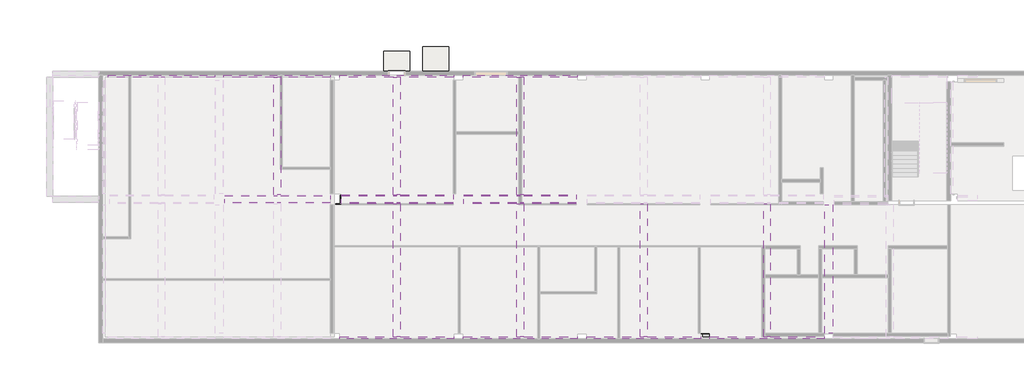
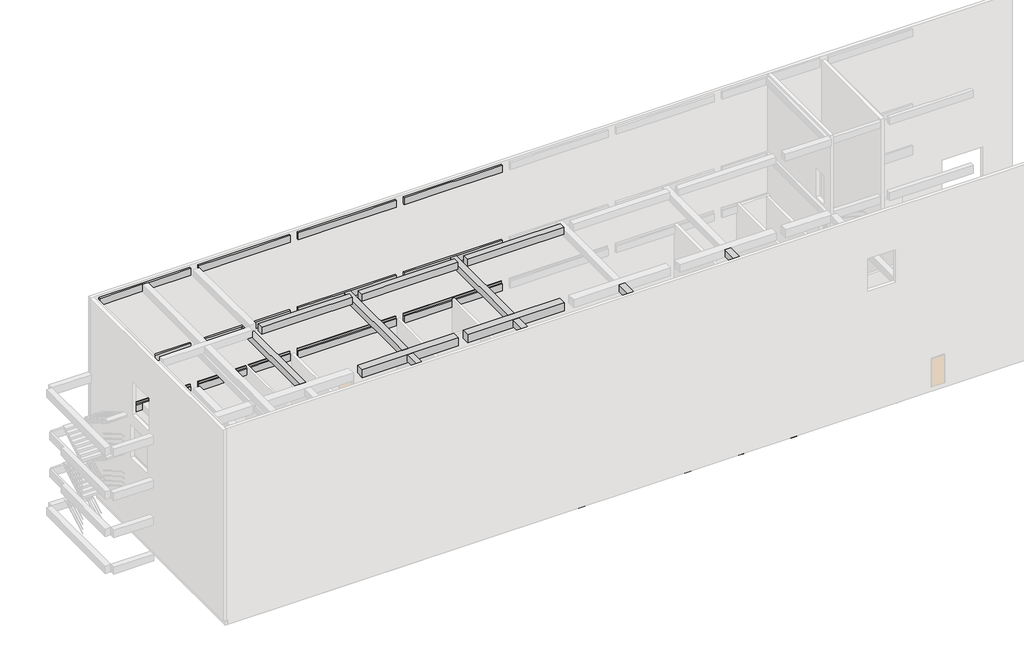
# One storey, part 3 of 5: 54 beams, 2 slabs.
# Revit data of these elements (continued)
# Room at (49621.297, 12708.408) mm, phase "New Construction", upper level "TOC", upper offset 9000 mm, lower offset 0 mm (continued)
#   H_Wall-Base Material-2 = ""
#   H_Wall-Base Material-3 = ""
#   H_Floor-Base Material-1 = "Concrete Slab"
#   H_Floor-Base Material-2 = ""
#   H_Floor-Base Material-3 = "Screed"
#   H_Floor-Base Material-4 = "Waterproof Membrane"
#   H_Floor-Base Material-5 = "Ceramic Tile"
#   H_Floor Finish-1 = "Ceramic Tile"
#   H_Floor Finish-2 = ""
#   H_Floor Finish Remark = ""
#   H_Skirt Base Material = "Same as Wall"
#   H_Skirt-Base Material-1 = ""
#   H_Skirt-Base Material-2 = ""
#   H_Skirt-Base Material-3 = ""
#   H_Skirt-Base Material-4 = ""
#   H_Skirt-Base Material-5 = ""
#   H_Skirt Finish-1 = "Acrylic Emulsion Paint"
#   H_Skirt Finish-2 = ""
#   H_Skirt Finish Remark = ""
#   H_Wall Finish Style Name = "Glazed Ceramic Tile (≤C.H+100) / No Paint (>C.H+100)"
#   H_Wall Base Material = "Masonry Wall / Waterproof Membrane"
#   H_Wall-Base Material-4 = "Waterproof Membrane"
#   H_Wall-Base Material-5 = "Glazed Ceramic Tile"
#   H_Wall Finish-1 = "Glazed Ceramic Tile"
#   H_Wall Finish-2 = ""
#   H_Wall Finish Remark = "Below Suspended Ceiling\nGlazed Ceramic Tile(≤C.H+100) + Waterproofing Membrane / No Paint (>C.H+100)"
#   H_Ceiling Finish Style Name = "Suspended Moisture Resistant Tiled Ceiling (T-Bar)"
#   H_Ceiling Base Material = "Concrete Slab / Fair Faced Concrete"
#   H_Ceiling-Base Material-1 = "(Concrete Slab)"
#   H_Ceiling-Base Material-2 = "(Fair Faced Concrete)"
#   H_Ceiling-Base Material-3 = ""
#   H_Ceiling-Base Material-4 = ""
#   H_Ceiling-Base Material-5 = "Moisture Resistant Tiled Ceiling System (T-Bar)"
#   H_Ceiling Finish-1 = "Moisture Resistant Tiled Ceiling System (T-Bar)"
#   H_Ceiling Finish-2 = ""
#   H_Ceiling Finish Remark = "600x600\nT bar"
#   H_Room W = 2700 mm
#   H_Room L = 1400 mm
#   H_Room H or CH = 9000 mm
#   Floor Finish Style No = none
#   Skirt Finish Style No = none
#   Wall Finish Style No = W32F
#   Ceiling Finish Style No = C96B
# Room at (52871.108, 13591.136) mm, phase "New Construction", upper level "TOC", upper offset 9000 mm, lower offset 0 mm
#   Comments = ""
#   Number = "110"
#   Name = "STAIRCASE"
#   H_Floor Finish Style Name = "Vinyl Tile"
#   H_Floor Base Material = "Concrete Slab / Steel Trowel Finish"
#   H_Wall-Base Material-1 = "Concrete Wall"
#   H_Skirt Finish Style Name = "Coved Vinyl Tile"
#   H_Wall-Base Material-2 = "(Fair Faced Concrete)"
#   H_Wall-Base Material-3 = ""
#   H_Floor-Base Material-1 = "Concrete Slab"
#   H_Floor-Base Material-2 = "Steel Trowel Finish"
#   H_Floor-Base Material-3 = ""
#   H_Floor-Base Material-4 = ""
#   H_Floor-Base Material-5 = "Vinyl Tile"
#   H_Floor Finish-1 = "Vinyl Tile"
#   H_Floor Finish-2 = ""
#   H_Floor Finish Remark = ""
#   H_Skirt Base Material = "Same as Wall"
#   H_Skirt-Base Material-1 = ""
#   H_Skirt-Base Material-2 = ""
#   H_Skirt-Base Material-3 = ""
#   H_Skirt-Base Material-4 = ""
#   H_Skirt-Base Material-5 = ""
#   H_Skirt Finish-1 = "Vinyl Tile"
#   H_Skirt Finish-2 = ""
#   H_Skirt Finish Remark = "Vinyl Tile = PVC Tile (polyvinyl chloride)"
#   H_Wall Finish Style Name = "Water Emulsion Paint"
#   H_Wall Base Material = "Concrete Wall / Fair Faced Concrete"
#   H_Wall-Base Material-4 = ""
#   H_Wall-Base Material-5 = ""
#   H_Wall Finish-1 = "Water Emulsion Paint"
#   H_Wall Finish-2 = ""
#   H_Wall Finish Remark = ""
#   H_Ceiling Finish Style Name = "Water Emulsion Paint"
#   H_Ceiling Base Material = "Concrete Slab / Fair Faced Concrete"
#   H_Ceiling-Base Material-1 = "(Concrete Slab)"
#   H_Ceiling-Base Material-2 = ""
#   H_Ceiling-Base Material-3 = ""
#   H_Ceiling-Base Material-4 = ""
#   H_Ceiling-Base Material-5 = ""
#   H_Ceiling Finish-1 = "Water Emulsion Paint"
#   H_Ceiling Finish-2 = ""
#   H_Ceiling Finish Remark = ""
#   H_Room W = 2000 mm
#   H_Room L = 8000 mm
#   H_Room H or CH = 9000 mm
#   Floor Finish Style No = none
#   Skirt Finish Style No = none
#   Wall Finish Style No = W02A
#   Ceiling Finish Style No = C02
# Room at (56962.839, 14779.531) mm, phase "New Construction", upper level "TOC", upper offset 9000 mm, lower offset 0 mm
#   Comments = ""
#   Number = "124"
#   Name = "F.O TANK ROOM"
#   H_Floor Finish Style Name = "Non-Slip Epoxy Paint"
#   H_Floor Base Material = "Concrete Slab / Steel Trowel Finish"
#   H_Wall-Base Material-1 = "Masonry Wall"
#   H_Skirt Finish Style Name = "Epoxy Paint"
#   H_Wall-Base Material-2 = ""
#   H_Wall-Base Material-3 = "Plastering"
#   H_Floor-Base Material-1 = "Concrete Slab"
#   H_Floor-Base Material-2 = "Steel Trowel Finish"
#   H_Floor-Base Material-3 = ""
#   H_Floor-Base Material-4 = ""
#   H_Floor-Base Material-5 = ""
#   H_Floor Finish-1 = "Epoxy Paint"
#   H_Floor Finish-2 = ""
#   H_Floor Finish Remark = "*WM 기준 확인 필요 Epoxy Paint \n(용제형, 0.1mm 이하) : epoxy resin + polyamine hardener(경화제)"
#   H_Skirt Base Material = "Same as Wall"
#   H_Skirt-Base Material-1 = ""
#   H_Skirt-Base Material-2 = ""
#   H_Skirt-Base Material-3 = ""
#   H_Skirt-Base Material-4 = ""
#   H_Skirt-Base Material-5 = ""
#   H_Skirt Finish-1 = "Epoxy Paint"
#   H_Skirt Finish-2 = ""
#   H_Skirt Finish Remark = "SACE"
#   H_Wall Finish Style Name = "Water Emulsion Paint"
#   H_Wall Base Material = "Masonry Wall / Cement Plaster"
#   H_Wall-Base Material-4 = ""
#   H_Wall-Base Material-5 = ""
#   H_Wall Finish-1 = ""
#   H_Wall Finish-2 = ""
#   H_Wall Finish Remark = ""
#   H_Ceiling Finish Style Name = "Water Emulsion Paint"
#   H_Ceiling Base Material = "Concrete Slab / Fair Faced Concrete"
#   H_Ceiling-Base Material-1 = "(Concrete Slab)"
#   H_Ceiling-Base Material-2 = ""
#   H_Ceiling-Base Material-3 = ""
#   H_Ceiling-Base Material-4 = ""
#   H_Ceiling-Base Material-5 = ""
#   H_Ceiling Finish-1 = "Water Emulsion Paint"
#   H_Ceiling Finish-2 = ""
#   H_Ceiling Finish Remark = ""
#   H_Room W = 3800 mm
#   H_Room L = 8400 mm
#   H_Room H or CH = 9000 mm
#   Floor Finish Style No = none
#   Skirt Finish Style No = none
#   Wall Finish Style No = W02B
#   Ceiling Finish Style No = C02
# Room at (61954.58, 4867.401) mm, phase "New Construction", upper level "TOC", upper offset 9000 mm, lower offset 0 mm
#   Comments = ""
#   Number = "125"
#   Name = "HVAC ROOM"
#   H_Floor Finish Style Name = "Non-Slip Epoxy Paint"
#   H_Floor Base Material = "Concrete Slab / Steel Trowel Finish"
#   H_Wall-Base Material-1 = "Masonry Wall"
#   H_Skirt Finish Style Name = "Epoxy Paint"
#   H_Wall-Base Material-2 = ""
#   H_Wall-Base Material-3 = "Plastering"
#   H_Floor-Base Material-1 = "Concrete Slab"
#   H_Floor-Base Material-2 = "Steel Trowel Finish"
#   H_Floor-Base Material-3 = ""
#   H_Floor-Base Material-4 = ""
#   H_Floor-Base Material-5 = ""
#   H_Floor Finish-1 = "Epoxy Paint"
#   H_Floor Finish-2 = ""
#   H_Floor Finish Remark = "*WM 기준 확인 필요 Epoxy Paint \n(용제형, 0.1mm 이하) : epoxy resin + polyamine hardener(경화제)"
#   H_Skirt Base Material = "Same as Wall"
#   H_Skirt-Base Material-1 = ""
#   H_Skirt-Base Material-2 = ""
#   H_Skirt-Base Material-3 = ""
#   H_Skirt-Base Material-4 = ""
#   H_Skirt-Base Material-5 = ""
#   H_Skirt Finish-1 = "Epoxy Paint"
#   H_Skirt Finish-2 = ""
#   H_Skirt Finish Remark = "SACE"
#   H_Wall Finish Style Name = "Water Emulsion Paint"
#   H_Wall Base Material = "Masonry Wall / Cement Plaster"
#   H_Wall-Base Material-4 = ""
#   H_Wall-Base Material-5 = ""
#   H_Wall Finish-1 = ""
#   H_Wall Finish-2 = ""
#   H_Wall Finish Remark = ""
#   H_Room W = 3600 mm
#   H_Room L = 4100 mm
#   H_Room H or CH = 9000 mm
#   Floor Finish Style No = none
#   Skirt Finish Style No = none
#   Wall Finish Style No = W02B
# Room at (52877.947, 3986.832) mm, phase "New Construction", upper level "TOC", upper offset 9000 mm, lower offset 0 mm
#   Comments = ""
#   Number = "122"
#   Name = "CYLINDER ROOM (HFC-23)"
#   H_Floor Finish Style Name = "Non-Slip Epoxy Paint"
#   H_Floor Base Material = "Concrete Slab / Steel Trowel Finish"
#   H_Wall-Base Material-1 = "Masonry Wall"
#   H_Skirt Finish Style Name = "Epoxy Paint"
#   H_Wall-Base Material-2 = ""
#   H_Wall-Base Material-3 = "Plastering"
#   H_Floor-Base Material-1 = "Concrete Slab"
#   H_Floor-Base Material-2 = "Steel Trowel Finish"
#   H_Floor-Base Material-3 = ""
#   H_Floor-Base Material-4 = ""
#   H_Floor-Base Material-5 = ""
#   H_Floor Finish-1 = "Epoxy Paint"
#   H_Floor Finish-2 = ""
#   H_Floor Finish Remark = "*WM 기준 확인 필요 Epoxy Paint \n(용제형, 0.1mm 이하) : epoxy resin + polyamine hardener(경화제)"
#   H_Skirt Base Material = "Same as Wall"
#   H_Skirt-Base Material-1 = ""
#   H_Skirt-Base Material-2 = ""
#   H_Skirt-Base Material-3 = ""
#   H_Skirt-Base Material-4 = ""
#   H_Skirt-Base Material-5 = ""
#   H_Skirt Finish-1 = "Epoxy Paint"
#   H_Skirt Finish-2 = ""
#   H_Skirt Finish Remark = "SACE"
#   H_Wall Finish Style Name = "Water Emulsion Paint"
#   H_Wall Base Material = "Masonry Wall / Cement Plaster"
#   H_Wall-Base Material-4 = ""
#   H_Wall-Base Material-5 = ""
#   H_Wall Finish-1 = ""
#   H_Wall Finish-2 = ""
#   H_Wall Finish Remark = ""
#   H_Ceiling Finish Style Name = "Water Emulsion Paint"
#   H_Ceiling Base Material = "Concrete Slab / Fair Faced Concrete"
#   H_Ceiling-Base Material-1 = "(Concrete Slab)"
#   H_Ceiling-Base Material-2 = ""
#   H_Ceiling-Base Material-3 = ""
#   H_Ceiling-Base Material-4 = ""
#   H_Ceiling-Base Material-5 = ""
#   H_Ceiling Finish-1 = "Water Emulsion Paint"
#   H_Ceiling Finish-2 = ""
#   H_Ceiling Finish Remark = ""
#   H_Room W = 14300 mm
#   H_Room L = 8900 mm
#   H_Room H or CH = 9000 mm
#   Floor Finish Style No = none
#   Skirt Finish Style No = none
#   Wall Finish Style No = W02B
#   Ceiling Finish Style No = C02
# Room at (47560.665, 5409.289) mm, phase "New Construction", upper level "TOC", upper offset 9000 mm, lower offset 0 mm
#   Comments = ""
#   Number = "119"
#   Name = "DISABLED TOILET(M)"
#   H_Floor Finish Style Name = "Non-Slip Unglazed Ceramic Tile"
#   H_Floor Base Material = "Concrete Slab / Screed / Liquid Waterproofing"
#   H_Wall-Base Material-1 = "Masonry Wall"
#   H_Wall-Base Material-2 = ""
#   H_Wall-Base Material-3 = ""
#   H_Floor-Base Material-1 = "Concrete Slab"
#   H_Floor-Base Material-2 = ""
#   H_Floor-Base Material-3 = "Screed"
#   H_Floor-Base Material-4 = "Liquid Waterproofing"
#   H_Floor-Base Material-5 = "Ceramic Tile"
#   H_Floor Finish-1 = "Ceramic Tile"
#   H_Floor Finish-2 = ""
#   H_Floor Finish Remark = ""
#   H_Wall Finish Style Name = "Glazed Ceramic Tile (≤C.H+100) / No Paint (>C.H+100)"
#   H_Wall Base Material = "Masonry Wall"
#   H_Wall-Base Material-4 = "No Waterproofing"
#   H_Wall-Base Material-5 = "Glazed Ceramic Tile"
#   H_Wall Finish-1 = "Glazed Ceramic Tile"
#   H_Wall Finish-2 = ""
#   H_Wall Finish Remark = "Below Suspended Ceiling\nGlazed Ceramic Tile(≤C.H+100) / No Paint (>C.H+100)"
#   H_Ceiling Finish Style Name = "Suspended Gypsum Plaster Board Ceiling (M-Bar)"
#   H_Ceiling Base Material = "Concrete Slab / Fair Faced Concrete"
#   H_Ceiling-Base Material-1 = "(Concrete Slab)"
#   H_Ceiling-Base Material-2 = "(Fair Faced Concrete)"
#   H_Ceiling-Base Material-3 = ""
#   H_Ceiling-Base Material-4 = ""
#   H_Ceiling-Base Material-5 = "Gypsum Plaster Board Ceiling System"
#   H_Ceiling Finish-1 = "Gypsum Plaster Board Ceiling System"
#   H_Ceiling Finish-2 = ""
#   H_Ceiling Finish Remark = ""
#   H_Room W = 4400 mm
#   H_Room L = 3700 mm
#   H_Room H or CH = 9000 mm
#   Floor Finish Style No = none
#   Wall Finish Style No = W32D
#   Ceiling Finish Style No = C92
# Room at (44106.126, 5206.081) mm, phase "New Construction", upper level "TOC", upper offset 9000 mm, lower offset 0 mm
#   Comments = ""
#   Number = "118"
#   Name = "DISABLED TOILET(W)"
#   H_Floor Finish Style Name = "Non-Slip Unglazed Ceramic Tile"
#   H_Floor Base Material = "Concrete Slab / Screed / Liquid Waterproofing"
#   H_Wall-Base Material-1 = "Masonry Wall"
#   H_Wall-Base Material-2 = ""
#   H_Wall-Base Material-3 = ""
#   H_Floor-Base Material-1 = "Concrete Slab"
#   H_Floor-Base Material-2 = ""
#   H_Floor-Base Material-3 = "Screed"
#   H_Floor-Base Material-4 = "Liquid Waterproofing"
#   H_Floor-Base Material-5 = "Ceramic Tile"
#   H_Floor Finish-1 = "Ceramic Tile"
#   H_Floor Finish-2 = ""
#   H_Floor Finish Remark = ""
#   H_Wall Finish Style Name = "Glazed Ceramic Tile (≤C.H+100) / No Paint (>C.H+100)"
#   H_Wall Base Material = "Masonry Wall"
#   H_Wall-Base Material-4 = "No Waterproofing"
#   H_Wall-Base Material-5 = "Glazed Ceramic Tile"
#   H_Wall Finish-1 = "Glazed Ceramic Tile"
#   H_Wall Finish-2 = ""
#   H_Wall Finish Remark = "Below Suspended Ceiling\nGlazed Ceramic Tile(≤C.H+100) / No Paint (>C.H+100)"
#   H_Ceiling Finish Style Name = "Suspended Gypsum Plaster Board Ceiling (M-Bar)"
#   H_Ceiling Base Material = "Concrete Slab / Fair Faced Concrete"
#   H_Ceiling-Base Material-1 = "(Concrete Slab)"
#   H_Ceiling-Base Material-2 = "(Fair Faced Concrete)"
#   H_Ceiling-Base Material-3 = ""
#   H_Ceiling-Base Material-4 = ""
#   H_Ceiling-Base Material-5 = "Gypsum Plaster Board Ceiling System"
#   H_Ceiling Finish-1 = "Gypsum Plaster Board Ceiling System"
#   H_Ceiling Finish-2 = ""
#   H_Ceiling Finish Remark = ""
#   H_Room W = 2300 mm
#   H_Room L = 1900 mm
#   H_Room H or CH = 9000 mm
#   Floor Finish Style No = none
#   Wall Finish Style No = W32D
#   Ceiling Finish Style No = C92
# Room at (44139.994, 3106.263) mm, phase "New Construction", upper level "TOC", upper offset 9000 mm, lower offset 0 mm
#   Comments = ""
#   Number = "120"
#   Name = "TOILET (W)"
#   H_Floor Finish Style Name = "Non-Slip Unglazed Ceramic Tile"
#   H_Floor Base Material = "Concrete Slab / Screed / Liquid Waterproofing"
#   H_Wall-Base Material-1 = "Masonry Wall"
#   H_Wall-Base Material-2 = ""
#   H_Wall-Base Material-3 = ""
#   H_Floor-Base Material-1 = "Concrete Slab"
#   H_Floor-Base Material-2 = ""
#   H_Floor-Base Material-3 = "Screed"
#   H_Floor-Base Material-4 = "Liquid Waterproofing"
#   H_Floor-Base Material-5 = "Ceramic Tile"
#   H_Floor Finish-1 = "Ceramic Tile"
#   H_Floor Finish-2 = ""
#   H_Floor Finish Remark = ""
#   H_Wall Finish Style Name = "Glazed Ceramic Tile (≤C.H+100) / No Paint (>C.H+100)"
#   H_Wall Base Material = "Masonry Wall"
#   H_Wall-Base Material-4 = "No Waterproofing"
#   H_Wall-Base Material-5 = "Glazed Ceramic Tile"
#   H_Wall Finish-1 = "Glazed Ceramic Tile"
#   H_Wall Finish-2 = ""
#   H_Wall Finish Remark = "Below Suspended Ceiling\nGlazed Ceramic Tile(≤C.H+100) / No Paint (>C.H+100)"
#   H_Ceiling Finish Style Name = "Suspended Gypsum Plaster Board Ceiling (M-Bar)"
#   H_Ceiling Base Material = "Concrete Slab / Fair Faced Concrete"
#   H_Ceiling-Base Material-1 = "(Concrete Slab)"
#   H_Ceiling-Base Material-2 = "(Fair Faced Concrete)"
#   H_Ceiling-Base Material-3 = ""
#   H_Ceiling-Base Material-4 = ""
#   H_Ceiling-Base Material-5 = "Gypsum Plaster Board Ceiling System"
#   H_Ceiling Finish-1 = "Gypsum Plaster Board Ceiling System"
#   H_Ceiling Finish-2 = ""
#   H_Ceiling Finish Remark = ""
#   H_Room W = 2300 mm
#   H_Room L = 1900 mm
#   H_Room H or CH = 9000 mm
#   Floor Finish Style No = none
#   Wall Finish Style No = W32D
#   Ceiling Finish Style No = C92
# Room at (36248.742, 3377.207) mm, phase "New Construction", upper level "TOC", upper offset 9000 mm, lower offset 0 mm
#   Comments = ""
#   Number = "116"
#   Name = "PRESIDENT ROOM"
#   H_Floor Finish Style Name = "Matwell"
#   H_Floor Base Material = "(기존 Floor Finish)"
#   H_Wall-Base Material-1 = "Masonry Wall"
#   H_Skirt Finish Style Name = "Coved Vinyl Tile"
#   H_Wall-Base Material-2 = ""
#   H_Wall-Base Material-3 = "Plastering"
#   H_Floor-Base Material-1 = "Recess Floor Mat"
#   H_Floor-Base Material-2 = ""
#   H_Floor-Base Material-3 = ""
#   H_Floor-Base Material-4 = ""
#   H_Floor-Base Material-5 = ""
#   H_Floor Finish-1 = ""
#   H_Floor Finish-2 = ""
#   H_Floor Finish Remark = "* 기존 Floor Finsh 위에 Mat 의 설치면적 만큼 별도의 Family 적용"
#   H_Skirt Base Material = "Same as Wall"
#   H_Skirt-Base Material-1 = ""
#   H_Skirt-Base Material-2 = ""
#   H_Skirt-Base Material-3 = ""
#   H_Skirt-Base Material-4 = ""
#   H_Skirt-Base Material-5 = ""
#   H_Skirt Finish-1 = "Vinyl Tile"
#   H_Skirt Finish-2 = ""
#   H_Skirt Finish Remark = "Vinyl Tile = PVC Tile (polyvinyl chloride)"
#   H_Wall Finish Style Name = "Water Emulsion Paint"
#   H_Wall Base Material = "Masonry Wall / Cement Plaster"
#   H_Wall-Base Material-4 = ""
#   H_Wall-Base Material-5 = ""
#   H_Wall Finish-1 = ""
#   H_Wall Finish-2 = ""
#   H_Wall Finish Remark = ""
#   H_Ceiling Finish Style Name = "Suspended Acoustic Tiled Ceiling (M-Bar)"
#   H_Ceiling Base Material = "Concrete Slab / Fair Faced Concrete"
#   H_Ceiling-Base Material-1 = "(Concrete Slab)"
#   H_Ceiling-Base Material-2 = "(Fair Faced Concrete)"
#   H_Ceiling-Base Material-3 = ""
#   H_Ceiling-Base Material-4 = ""
#   H_Ceiling-Base Material-5 = "Acoustic Tiled Ceiling System (M-Bar)"
#   H_Ceiling Finish-1 = "Acoustic Tiled Ceiling System (M-Bar)"
#   H_Ceiling Finish-2 = ""
#   H_Ceiling Finish Remark = ""
#   H_Room W = 8000 mm
#   H_Room L = 6100 mm
#   H_Room H or CH = 9000 mm
#   Floor Finish Style No = none
#   Skirt Finish Style No = none
#   Wall Finish Style No = W02B
#   Ceiling Finish Style No = C95A
# Room at (30050.892, 2259.562) mm, phase "New Construction", upper level "TOC", upper offset 9000 mm, lower offset 0 mm
#   Comments = ""
#   Number = "114"
#   Name = "STORAGE"
#   H_Floor Finish Style Name = "Vinyl Tile"
#   H_Floor Base Material = "Concrete Slab / Steel Trowel Finish"
#   H_Wall-Base Material-1 = "Masonry Wall"
#   H_Skirt Finish Style Name = "Coved Vinyl Tile"
#   H_Wall-Base Material-2 = ""
#   H_Wall-Base Material-3 = "Plastering"
#   H_Floor-Base Material-1 = "Concrete Slab"
#   H_Floor-Base Material-2 = "Steel Trowel Finish"
#   H_Floor-Base Material-3 = ""
#   H_Floor-Base Material-4 = ""
#   H_Floor-Base Material-5 = "Vinyl Tile"
#   H_Floor Finish-1 = "Vinyl Tile"
#   H_Floor Finish-2 = ""
#   H_Floor Finish Remark = ""
#   H_Skirt Base Material = "Same as Wall"
#   H_Skirt-Base Material-1 = ""
#   H_Skirt-Base Material-2 = ""
#   H_Skirt-Base Material-3 = ""
#   H_Skirt-Base Material-4 = ""
#   H_Skirt-Base Material-5 = ""
#   H_Skirt Finish-1 = "Vinyl Tile"
#   H_Skirt Finish-2 = ""
#   H_Skirt Finish Remark = "Vinyl Tile = PVC Tile (polyvinyl chloride)"
#   H_Wall Finish Style Name = "Water Emulsion Paint"
#   H_Wall Base Material = "Masonry Wall / Cement Plaster"
#   H_Wall-Base Material-4 = ""
#   H_Wall-Base Material-5 = ""
#   H_Wall Finish-1 = ""
#   H_Wall Finish-2 = ""
#   H_Wall Finish Remark = ""
#   H_Ceiling Finish Style Name = "Suspended Gypsum Plaster Board Ceiling (M-Bar)"
#   H_Ceiling Base Material = "Concrete Slab / Fair Faced Concrete"
#   H_Ceiling-Base Material-1 = "(Concrete Slab)"
#   H_Ceiling-Base Material-2 = "(Fair Faced Concrete)"
#   H_Ceiling-Base Material-3 = ""
#   H_Ceiling-Base Material-4 = ""
#   H_Ceiling-Base Material-5 = "Gypsum Plaster Board Ceiling System"
#   H_Ceiling Finish-1 = "Gypsum Plaster Board Ceiling System"
#   H_Ceiling Finish-2 = ""
#   H_Ceiling Finish Remark = ""
#   H_Room W = 5200 mm
#   H_Room L = 6100 mm
#   H_Room H or CH = 9000 mm
#   Floor Finish Style No = none
#   Skirt Finish Style No = none
#   Wall Finish Style No = W02B
#   Ceiling Finish Style No = C92
# Room at (30017.024, 4901.269) mm, phase "New Construction", upper level "TOC", upper offset 9000 mm, lower offset 0 mm
#   Comments = ""
#   Number = "113"
#   Name = "MAAMS REST ROOM"
#   H_Floor Finish Style Name = "Vinyl Tile"
#   H_Floor Base Material = "Concrete Slab / Steel Trowel Finish"
#   H_Wall-Base Material-1 = "Masonry Wall"
#   H_Skirt Finish Style Name = "Coved Vinyl Tile"
#   H_Wall-Base Material-2 = ""
#   H_Wall-Base Material-3 = "Plastering"
#   H_Floor-Base Material-1 = "Concrete Slab"
#   H_Floor-Base Material-2 = "Steel Trowel Finish"
#   H_Floor-Base Material-3 = ""
#   H_Floor-Base Material-4 = ""
#   H_Floor-Base Material-5 = "Vinyl Tile"
#   H_Floor Finish-1 = "Vinyl Tile"
#   H_Floor Finish-2 = ""
#   H_Floor Finish Remark = ""
#   H_Skirt Base Material = "Same as Wall"
#   H_Skirt-Base Material-1 = ""
#   H_Skirt-Base Material-2 = ""
#   H_Skirt-Base Material-3 = ""
#   H_Skirt-Base Material-4 = ""
#   H_Skirt-Base Material-5 = ""
#   H_Skirt Finish-1 = "Vinyl Tile"
#   H_Skirt Finish-2 = ""
#   H_Skirt Finish Remark = "Vinyl Tile = PVC Tile (polyvinyl chloride)"
#   H_Wall Finish Style Name = "Water Emulsion Paint"
#   H_Wall Base Material = "Masonry Wall / Cement Plaster"
#   H_Wall-Base Material-4 = ""
#   H_Wall-Base Material-5 = ""
#   H_Wall Finish-1 = ""
#   H_Wall Finish-2 = ""
#   H_Wall Finish Remark = ""
#   H_Ceiling Finish Style Name = "Suspended Gypsum Plaster Board Ceiling (M-Bar)"
#   H_Ceiling Base Material = "Concrete Slab / Fair Faced Concrete"
#   H_Ceiling-Base Material-1 = "(Concrete Slab)"
#   H_Ceiling-Base Material-2 = "(Fair Faced Concrete)"
#   H_Ceiling-Base Material-3 = ""
#   H_Ceiling-Base Material-4 = ""
#   H_Ceiling-Base Material-5 = "Gypsum Plaster Board Ceiling System"
#   H_Ceiling Finish-1 = "Gypsum Plaster Board Ceiling System"
#   H_Ceiling Finish-2 = ""
#   H_Ceiling Finish Remark = ""
#   H_Room W = 5200 mm
#   H_Room L = 6100 mm
#   H_Room H or CH = 9000 mm
#   Floor Finish Style No = none
#   Skirt Finish Style No = none
#   Wall Finish Style No = W02B
#   Ceiling Finish Style No = C92
# Room at (19246.99, 3580.415) mm, phase "New Construction", upper level "TOC", upper offset 9000 mm, lower offset 0 mm
#   Comments = ""
#   Number = "112"
#   Name = "CONFERENCE ROOM"
#   H_Floor Finish Style Name = "Matwell"
#   H_Floor Base Material = "(기존 Floor Finish)"
#   H_Wall-Base Material-1 = "Masonry Wall"
#   H_Skirt Finish Style Name = "Coved Vinyl Tile"
#   H_Wall-Base Material-2 = ""
#   H_Wall-Base Material-3 = "Plastering"
#   H_Floor-Base Material-1 = "Recess Floor Mat"
#   H_Floor-Base Material-2 = ""
#   H_Floor-Base Material-3 = ""
#   H_Floor-Base Material-4 = ""
#   H_Floor-Base Material-5 = ""
#   H_Floor Finish-1 = ""
#   H_Floor Finish-2 = ""
#   H_Floor Finish Remark = "* 기존 Floor Finsh 위에 Mat 의 설치면적 만큼 별도의 Family 적용"
#   H_Skirt Base Material = "Same as Wall"
#   H_Skirt-Base Material-1 = ""
#   H_Skirt-Base Material-2 = ""
#   H_Skirt-Base Material-3 = ""
#   H_Skirt-Base Material-4 = ""
#   H_Skirt-Base Material-5 = ""
#   H_Skirt Finish-1 = "Vinyl Tile"
#   H_Skirt Finish-2 = ""
#   H_Skirt Finish Remark = "Vinyl Tile = PVC Tile (polyvinyl chloride)"
#   H_Wall Finish Style Name = "Water Emulsion Paint"
#   H_Wall Base Material = "Masonry Wall / Cement Plaster"
#   H_Wall-Base Material-4 = ""
#   H_Wall-Base Material-5 = ""
#   H_Wall Finish-1 = ""
#   H_Wall Finish-2 = ""
#   H_Wall Finish Remark = ""
#   H_Ceiling Finish Style Name = "Suspended Acoustic Tiled Ceiling (M-Bar)"
#   H_Ceiling Base Material = "Concrete Slab / Fair Faced Concrete"
#   H_Ceiling-Base Material-1 = "(Concrete Slab)"
#   H_Ceiling-Base Material-2 = "(Fair Faced Concrete)"
#   H_Ceiling-Base Material-3 = ""
#   H_Ceiling-Base Material-4 = ""
#   H_Ceiling-Base Material-5 = "Acoustic Tiled Ceiling System (M-Bar)"
#   H_Ceiling Finish-1 = "Acoustic Tiled Ceiling System (M-Bar)"
#   H_Ceiling Finish-2 = ""
#   H_Ceiling Finish Remark = ""
#   H_Room W = 5100 mm
#   H_Room L = 6100 mm
#   H_Room H or CH = 9000 mm
#   Floor Finish Style No = none
#   Skirt Finish Style No = none
#   Wall Finish Style No = W02B
#   Ceiling Finish Style No = C95A
# Room at (61369.572, 13806.461) mm, phase "New Construction", upper level "TOC", upper offset 9000 mm, lower offset 0 mm
#   Comments = ""
#   Number = "123"
#   Name = "EDG ROOM"
#   H_Floor Finish Style Name = "Non-Slip Epoxy Paint"
#   H_Floor Base Material = "Concrete Slab / Steel Trowel Finish"
#   H_Wall-Base Material-1 = "Masonry Wall"
#   H_Skirt Finish Style Name = "Epoxy Paint"
#   H_Wall-Base Material-2 = ""
#   H_Wall-Base Material-3 = "Plastering"
#   H_Floor-Base Material-1 = "Concrete Slab"
#   H_Floor-Base Material-2 = "Steel Trowel Finish"
#   H_Floor-Base Material-3 = ""
#   H_Floor-Base Material-4 = ""
#   H_Floor-Base Material-5 = ""
#   H_Floor Finish-1 = "Epoxy Paint"
#   H_Floor Finish-2 = ""
#   H_Floor Finish Remark = "*WM 기준 확인 필요 Epoxy Paint \n(용제형, 0.1mm 이하) : epoxy resin + polyamine hardener(경화제)"
#   H_Skirt Base Material = "Same as Wall"
#   H_Skirt-Base Material-1 = ""
#   H_Skirt-Base Material-2 = ""
#   H_Skirt-Base Material-3 = ""
#   H_Skirt-Base Material-4 = ""
#   H_Skirt-Base Material-5 = ""
#   H_Skirt Finish-1 = "Epoxy Paint"
#   H_Skirt Finish-2 = ""
#   H_Skirt Finish Remark = "SACE"
#   H_Wall Finish Style Name = "Water Emulsion Paint"
#   H_Wall Base Material = "Masonry Wall / Cement Plaster"
#   H_Wall-Base Material-4 = ""
#   H_Wall-Base Material-5 = ""
#   H_Wall Finish-1 = ""
#   H_Wall Finish-2 = ""
#   H_Wall Finish Remark = ""
#   H_Ceiling Finish Style Name = "Water Emulsion Paint"
#   H_Ceiling Base Material = "Concrete Slab / Fair Faced Concrete"
#   H_Ceiling-Base Material-1 = "(Concrete Slab)"
#   H_Ceiling-Base Material-2 = ""
#   H_Ceiling-Base Material-3 = ""
#   H_Ceiling-Base Material-4 = ""
#   H_Ceiling-Base Material-5 = ""
#   H_Ceiling Finish-1 = "Water Emulsion Paint"
#   H_Ceiling Finish-2 = ""
#   H_Ceiling Finish Remark = ""
#   H_Room W = 8200 mm
#   H_Room L = 6100 mm
#   H_Room H or CH = 9000 mm
#   Floor Finish Style No = none
#   Skirt Finish Style No = none
#   Wall Finish Style No = W02B
#   Ceiling Finish Style No = C02
# Room at (33987.4, 7910.137) mm, phase "New Construction", upper level "TOC", upper offset 9000 mm, lower offset 0 mm
#   Comments = ""
#   Number = "111"
#   Name = "CORRIDOR"
#   H_Floor Finish Style Name = "Vinyl Tile"
#   H_Floor Base Material = "Concrete Slab / Steel Trowel Finish"
#   H_Wall-Base Material-1 = "Masonry Wall"
#   H_Skirt Finish Style Name = "Coved Vinyl Tile"
#   H_Wall-Base Material-2 = ""
#   H_Wall-Base Material-3 = "Plastering"
#   H_Floor-Base Material-1 = "Concrete Slab"
#   H_Floor-Base Material-2 = "Steel Trowel Finish"
#   H_Floor-Base Material-3 = ""
#   H_Floor-Base Material-4 = ""
#   H_Floor-Base Material-5 = "Vinyl Tile"
#   H_Floor Finish-1 = "Vinyl Tile"
#   H_Floor Finish-2 = ""
#   H_Floor Finish Remark = ""
#   H_Skirt Base Material = "Same as Wall"
#   H_Skirt-Base Material-1 = ""
#   H_Skirt-Base Material-2 = ""
#   H_Skirt-Base Material-3 = ""
#   H_Skirt-Base Material-4 = ""
#   H_Skirt-Base Material-5 = ""
#   H_Skirt Finish-1 = "Vinyl Tile"
#   H_Skirt Finish-2 = ""
#   H_Skirt Finish Remark = "Vinyl Tile = PVC Tile (polyvinyl chloride)"
#   H_Wall Finish Style Name = "Water Emulsion Paint"
#   H_Wall Base Material = "Masonry Wall / Cement Plaster"
#   H_Wall-Base Material-4 = ""
#   H_Wall-Base Material-5 = ""
#   H_Wall Finish-1 = ""
#   H_Wall Finish-2 = ""
#   H_Wall Finish Remark = ""
#   H_Ceiling Finish Style Name = "Suspended Gypsum Plaster Board Ceiling (M-Bar)"
#   H_Ceiling Base Material = "Concrete Slab / Fair Faced Concrete"
#   H_Ceiling-Base Material-1 = "(Concrete Slab)"
#   H_Ceiling-Base Material-2 = "(Fair Faced Concrete)"
#   H_Ceiling-Base Material-3 = ""
#   H_Ceiling-Base Material-4 = ""
#   H_Ceiling-Base Material-5 = "Gypsum Plaster Board Ceiling System"
#   H_Ceiling Finish-1 = "Gypsum Plaster Board Ceiling System"
#   H_Ceiling Finish-2 = ""
#   H_Ceiling Finish Remark = ""
#   H_Room W = 14400 mm
#   H_Room L = 8400 mm
#   H_Room H or CH = 9000 mm
#   Floor Finish Style No = none
#   Skirt Finish Style No = none
#   Wall Finish Style No = W02B
#   Ceiling Finish Style No = C92
